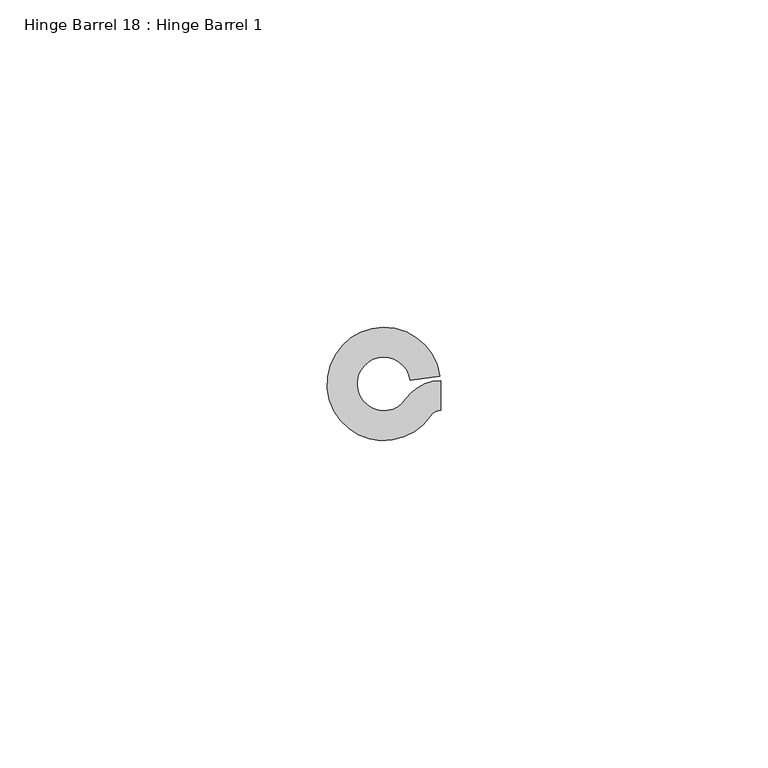
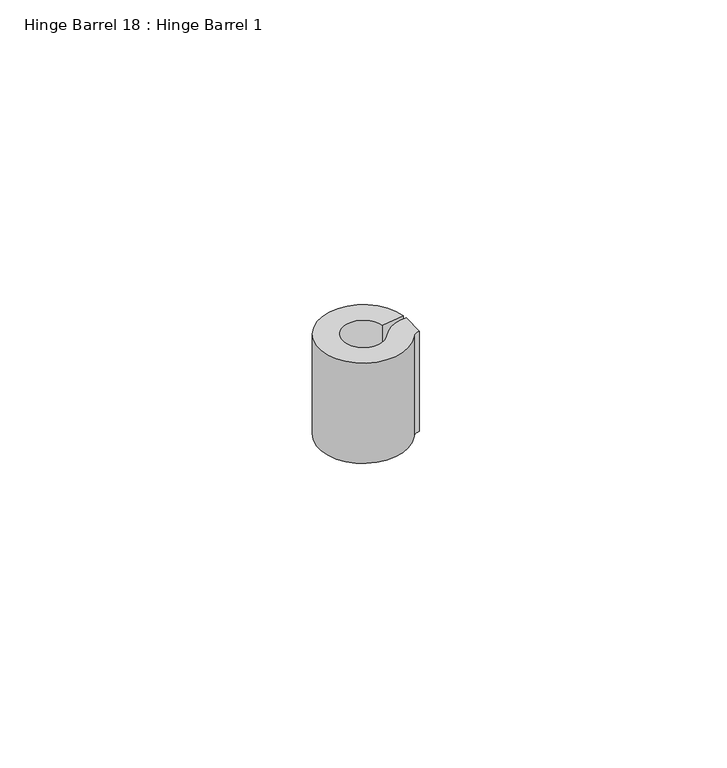
"""IFC4 building model written with IfcOpenShell, lengths in millimetres: proxy geometry, Hinge Barrel 18 : Hinge Barrel 1."""

from ifc_helpers import new_model, si_unit, point, frame, frame_2d, origin, place, context, project, spatial, polyline, circle_curve, trimmed, segment, composite_curve, outline, extrude, source, transform, mapped, element, save


def hinge_barrel_18_hinge_barrel_1_c85a10a0(model_context):
    return source(origin(), model_context, "Body", "SweptSolid", [
        extrude(outline(composite_curve([segment(trimmed(circle_curve(frame_2d((587327.8245257, -533990.5568067)), 6.4044851), [point((587322.5194669, -533986.9688017))], [point((587327.8245257, -533984.1523216))], False, "CARTESIAN"), True, "CONTINUOUS"), segment(polyline([(587327.8245257, -533984.1523216), (587327.8245257, -533988.7163841)]), True, "CONTINUOUS"), segment(trimmed(circle_curve(frame_2d((587327.8245257, -533990.5568067)), 1.8404226), [point((587327.8245257, -533988.7163841))], [point((587326.3000393, -533989.5257409))], True, "CARTESIAN"), True, "CONTINUOUS"), segment(trimmed(circle_curve(frame_2d((587319.1320739, -533984.6777841)), 8.6534625), [point((587326.3000393, -533989.5257409))], [point((587327.7022899, -533983.4803654))], False, "CARTESIAN"), True, "CONTINUOUS"), segment(polyline([(587327.7022899, -533983.4803654), (587323.1821338, -533984.1119153)]), True, "CONTINUOUS"), segment(trimmed(circle_curve(frame_2d((587319.1320739, -533984.6777841)), 4.0894), [point((587323.1821338, -533984.1119153))], [point((587322.5194669, -533986.9688017))], True, "CARTESIAN"), True, "CONTINUOUS")], self_intersect=False)), frame((0.0, 0.0, 438.15), z_axis=(0.0, 0.0, 1.0), x_axis=(1.0, 0.0, 0.0)), (0.0, 0.0, 1.0), 20.8359375),
    ])


if __name__ == "__main__":
    model = new_model("IFC4")
    model_context = context("Model", 3, world=origin())
    ifc_project = project(units=[si_unit("LENGTHUNIT", "METRE", prefix="MILLI")], contexts=[model_context])
    site = spatial("IfcSite", under=ifc_project)
    building = spatial("IfcBuilding", under=site)
    placement = place(None, origin())
    hinge_barrel_18_hinge_barrel_1_shape = hinge_barrel_18_hinge_barrel_1_c85a10a0(model_context)
    element("IfcBuildingElementProxy", 1, Name="Hinge Barrel 18 : Hinge Barrel 1", ObjectType="Hinge Barrel 18 : Hinge Barrel 1", at=placement, inside=building, context=model_context, shape_type="MappedRepresentation", body=[
        mapped(hinge_barrel_18_hinge_barrel_1_shape, transform((0.0, 0.0, 0.0), x_axis=(1.0, 0.0, 0.0), y_axis=(0.0, 1.0, 0.0), z_axis=(0.0, 0.0, 1.0))),
    ])
    save(model, "model.ifc")

# Revit data of these elements
# Element 1 (IfcBuildingElementProxy, "Hinge Barrel 18 : Hinge Barrel 1")
#   Materials on its faces: "6\"X6\" WELD-ON STL BUTT HINGE"
# Materials
#   "6\"X6\" WELD-ON STL BUTT HINGE": class "Metal", colour RGB 189 187 185, transparency 0, Description = "Carbon steel", Cost = 0
